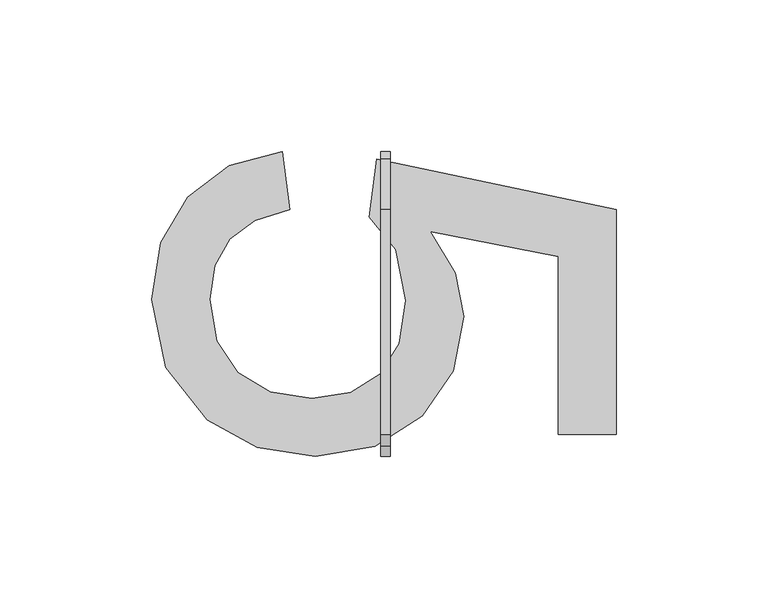
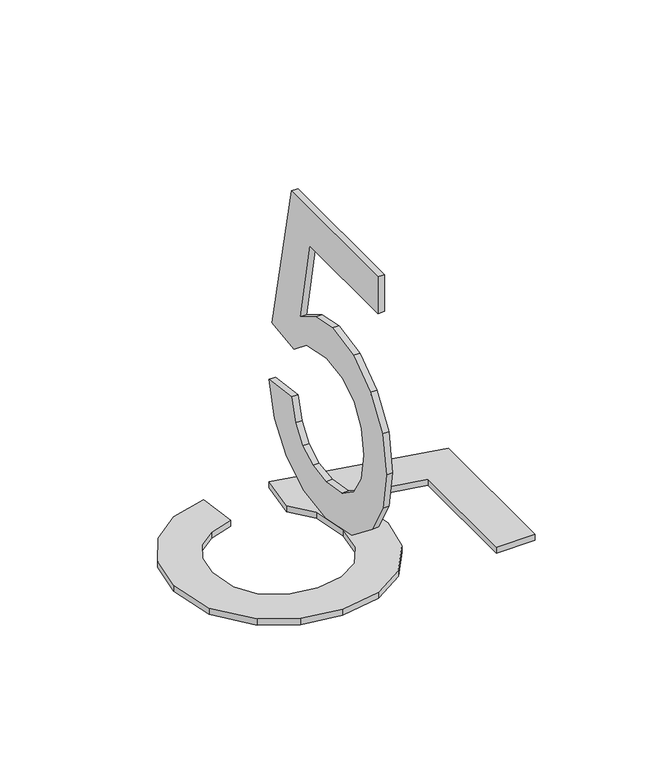
"""IFC4 building model written with IfcOpenShell, lengths in millimetres: proxy geometry, Grid Number2_FedEx : Grid Number2_FedEx."""

from ifc_helpers import new_model, si_unit, frame, origin, origin_with_axes, place, context, project, spatial, polyline, outline, extrude, source, transform, mapped, element, save


def entourage_214aeef9(model_context):
    return source(origin(), model_context, "Body", "SweptSolid", [
        extrude(outline(polyline([(-143.6079567, 271.5590522), (-141.2158408, 252.4221251), (-152.704538, 248.9087049), (-160.9321084, 242.7789079), (-165.8798638, 234.0607668), (-167.5291155, 222.7823142), (-165.2351138, 209.0650247), (-158.3531085, 198.7864017), (-147.677357, 192.3669345), (-134.0021163, 190.2271121), (-121.125805, 192.2314435), (-111.2770154, 198.244438), (-105.0257438, 208.3128164), (-102.9419866, 222.4832997), (-106.2685228, 239.2841761), (-114.9025661, 250.0300092), (-112.5104502, 269.1669363), (-33.570626, 252.4221251), (-33.570626, 178.2665326), (-52.707553, 178.2665326), (-52.707553, 236.9481255), (-94.8685955, 245.133647), (-86.5709435, 231.4630785), (-83.8050595, 217.1384158), (-87.2343819, 199.258284), (-97.5223491, 184.415018), (-113.2019212, 174.4213932), (-132.8060584, 171.090185), (-151.9429855, 174.089674), (-168.3140286, 183.0881412), (-182.0780391, 200.318851), (-186.6660426, 222.8570678), (-183.7179467, 241.6529315), (-174.8736588, 256.6270163), (-161.1610414, 266.8916229), (-143.6079567, 271.5590522)])), origin_with_axes(), (0.0, 0.0, 1.0), 3.175),
        extrude(outline(polyline([(271.5590522, 54.9042454), (266.8916229, 37.3511606), (256.6270163, 23.6385432), (241.6529315, 14.7942554), (222.8570678, 11.8461594), (200.318851, 16.4341629), (183.0881412, 30.1981735), (174.089674, 46.5692166), (171.090185, 65.7061437), (174.4213932, 85.3102809), (184.415018, 100.989853), (199.258284, 111.2778201), (217.1384158, 114.7071425), (231.4630785, 111.9412585), (245.133647, 103.6436065), (236.9481255, 145.804649), (178.2665326, 145.804649), (178.2665326, 164.9415761), (252.4221251, 164.9415761), (269.1669363, 86.0017519), (250.0300092, 83.609636), (239.2841761, 92.2436793), (222.4832997, 95.5702154), (208.3128164, 93.4864582), (198.244438, 87.2351866), (192.2314435, 77.386397), (190.2271121, 64.5100857), (192.3669345, 50.8348451), (198.7864017, 40.1590935), (209.0650247, 33.2770883), (222.7823142, 30.9830865), (234.0607668, 32.6323383), (242.7789079, 37.5800936), (248.9087049, 45.8076641), (252.4221251, 57.2963612), (271.5590522, 54.9042454)])), frame((-111.2489267, 0.0, 0.0), z_axis=(1.0, 0.0, 0.0), x_axis=(0.0, 1.0, 0.0)), (0.0, 0.0, 1.0), 3.175),
    ])


if __name__ == "__main__":
    model = new_model("IFC4")
    model_context = context("Model", 3, world=origin())
    ifc_project = project(units=[si_unit("LENGTHUNIT", "METRE", prefix="MILLI")], contexts=[model_context])
    site = spatial("IfcSite", under=ifc_project)
    building = spatial("IfcBuilding", under=site)
    placement = place(None, origin())
    entourage_shape = entourage_214aeef9(model_context)
    element("IfcBuildingElementProxy", 1, Name="Grid Number2_FedEx : Grid Number2_FedEx", ObjectType="Grid Number2_FedEx : Grid Number2_FedEx", at=placement, inside=building, context=model_context, shape_type="MappedRepresentation", body=[
        mapped(entourage_shape, transform((0.0, 0.0, 0.0), x_axis=(1.0, 0.0, 0.0), y_axis=(0.0, 1.0, 0.0), z_axis=(0.0, 0.0, 1.0))),
    ])
    save(model, "model.ifc")

# Revit data of these elements
# Type "Grid Number2_FedEx : Grid Number2_FedEx"
#   Grid [instance default] = "S"
#   Label Width [instance default] = 1' - 0"
#   Half Box Width2 [instance default] = 0' - 6.13846"
#   Half Box Width [instance default] = 0' - 6"
#   Robust [instance default] = yes
#   Height = 0
#   Assembly Code = ""
# Element 1 (IfcBuildingElementProxy, "Grid Number2_FedEx : Grid Number2_FedEx")
#   Grid = "5"
#   Robust = no
#   Materials on its faces: "Letter"
# Materials
#   "Letter": class "Unassigned", colour RGB 178 187 30, transparency 0, Comments = "Rendering appearance not upgraded "
